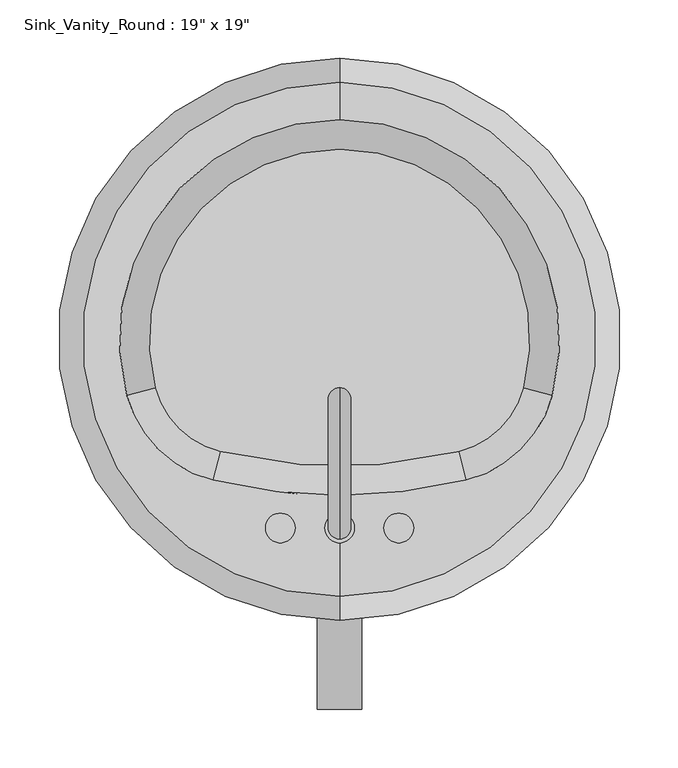
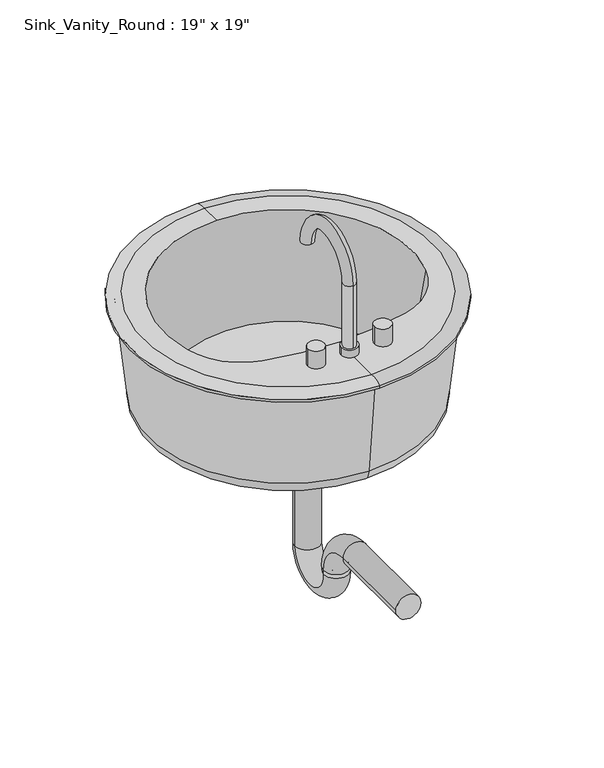
"""IFC4 building model written with IfcOpenShell, lengths in millimetres: flow terminal geometry."""

import ifcopenshell
import ifcopenshell.guid

model = None  # the IFC model being written
_history = None  # IfcOwnerHistory: only IFC2X3 demands one
_inside = {}  # id of a spatial element -> (the spatial element, [elements in it])
_under = {}  # id of a project, library or spatial element -> (it, [spatial elements below it])
_declared = {}  # id of a project -> (the project, [libraries it declares])
_typed = {}  # id of a type object -> (the type object, [elements of that type])
_made_of = {}  # id of a material, layer set ... -> (it, [elements and type objects made of it])


def new_model(schema):
    """Start an empty IFC model of exactly this schema.

    Asked for "IFC4X3", IfcOpenShell would pick the latest addendum, in which some entities
    have other attributes; the version numbers below select the first issue.
    IFC2X3 requires an IfcOwnerHistory on every rooted entity: one is made here for all.
    """
    global model, _history
    if schema == "IFC4X3":
        model = ifcopenshell.file(schema_version=(4, 3, 0, 0))
    else:
        model = ifcopenshell.file(schema=schema)
    _inside.clear()
    _under.clear()
    _declared.clear()
    _typed.clear()
    _made_of.clear()
    _history = None
    if model.schema == "IFC2X3":
        org = make("IfcOrganization", Name="unknown")
        user = make(
            "IfcPersonAndOrganization",
            ThePerson=make("IfcPerson", FamilyName="unknown"),
            TheOrganization=org,
        )
        app = make(
            "IfcApplication",
            ApplicationDeveloper=org,
            Version="unknown",
            ApplicationFullName="unknown",
            ApplicationIdentifier="unknown",
        )
        _history = make(
            "IfcOwnerHistory",
            OwningUser=user,
            OwningApplication=app,
            ChangeAction="ADDED",
            CreationDate=0,
        )
    return model


def make(cls, **values):
    """One entity of the class cls with the attributes given. An attribute that is None is left unset."""
    return model.create_entity(
        cls, **{name: value for name, value in values.items() if value is not None}
    )


def rooted(cls, **values):
    """An entity with a GlobalId (a new one), such as an element, a storey or a relation."""
    return make(cls, GlobalId=ifcopenshell.guid.new(), OwnerHistory=_history, **values)


def si_unit(unit_type, name, prefix=None):
    """IfcSIUnit, for example si_unit("LENGTHUNIT", "METRE", prefix="MILLI")."""
    return make("IfcSIUnit", UnitType=unit_type, Prefix=prefix, Name=name)


def assignment(units):
    """IfcUnitAssignment: the units of a project."""
    return None if units is None else make("IfcUnitAssignment", Units=units)


def point(xyz):
    """IfcCartesianPoint."""
    return None if xyz is None else make("IfcCartesianPoint", Coordinates=xyz)


def direction(xyz):
    """IfcDirection."""
    return None if xyz is None else make("IfcDirection", DirectionRatios=xyz)


def frame(location, z_axis=None, x_axis=None):
    """IfcAxis2Placement3D, a coordinate frame: its origin and axes. An axis left out is left unset."""
    return make(
        "IfcAxis2Placement3D",
        Location=point(location),
        Axis=direction(z_axis),
        RefDirection=direction(x_axis),
    )


def frame_2d(location, x_axis=None):
    """IfcAxis2Placement2D, a coordinate frame in the plane: its origin and x axis."""
    return make(
        "IfcAxis2Placement2D", Location=point(location), RefDirection=direction(x_axis)
    )


def origin():
    """The frame at (0, 0, 0) with its axes left unset."""
    return frame((0.0, 0.0, 0.0))


def place(relative_to, where):
    """IfcLocalPlacement: puts the frame where relative to a parent placement (None: the world)."""
    return make(
        "IfcLocalPlacement", PlacementRelTo=relative_to, RelativePlacement=where
    )


def context(
    kind, dimensions, precision=None, world=None, true_north=None, identifier=None
):
    """IfcGeometricRepresentationContext, for example the 3D "Model" context."""
    return make(
        "IfcGeometricRepresentationContext",
        ContextIdentifier=identifier,
        ContextType=kind,
        CoordinateSpaceDimension=dimensions,
        Precision=precision,
        WorldCoordinateSystem=world,
        TrueNorth=true_north,
    )


def project(units=None, contexts=None):
    """IfcProject with its units and contexts."""
    return rooted(
        "IfcProject",
        Name="project",
        RepresentationContexts=contexts,
        UnitsInContext=assignment(units),
    )


def spatial(cls, under=None, at=None, **own):
    """A site, building, storey or space (cls), placed at a placement, below another one or the project."""
    s = rooted(cls, ObjectPlacement=at, **own)
    if under is not None:
        _under.setdefault(under.id(), (under, []))[1].append(s)
    return s


def polyline(points):
    """IfcPolyline through the points."""
    return make("IfcPolyline", Points=[point(p) for p in points])


def circle_curve(where, radius):
    """IfcCircle in the frame where."""
    return make("IfcCircle", Position=where, Radius=radius)


def ellipse_curve(where, semi_axis1, semi_axis2):
    """IfcEllipse in the frame where."""
    return make(
        "IfcEllipse", Position=where, SemiAxis1=semi_axis1, SemiAxis2=semi_axis2
    )


def trimmed(basis, trim1, trim2, sense, master):
    """IfcTrimmedCurve: the piece of a basis curve between two trims."""
    return make(
        "IfcTrimmedCurve",
        BasisCurve=basis,
        Trim1=trim1,
        Trim2=trim2,
        SenseAgreement=sense,
        MasterRepresentation=master,
    )


def segment(curve, same_sense, transition):
    """IfcCompositeCurveSegment."""
    return make(
        "IfcCompositeCurveSegment",
        Transition=transition,
        SameSense=same_sense,
        ParentCurve=curve,
    )


def composite_curve(segments, self_intersect=None):
    """IfcCompositeCurve: segments joined end to end."""
    return make("IfcCompositeCurve", Segments=segments, SelfIntersect=self_intersect)


def outline(outer, holes=None, kind="AREA"):
    """IfcArbitraryClosedProfileDef: a profile drawn as a closed curve; with holes, ...WithVoids."""
    if holes is None:
        return make("IfcArbitraryClosedProfileDef", ProfileType=kind, OuterCurve=outer)
    return make(
        "IfcArbitraryProfileDefWithVoids",
        ProfileType=kind,
        OuterCurve=outer,
        InnerCurves=holes,
    )


def extrude(swept, where, along, depth):
    """IfcExtrudedAreaSolid: the profile swept, set in the frame where, extruded along a direction by depth."""
    return make(
        "IfcExtrudedAreaSolid",
        SweptArea=swept,
        Position=where,
        ExtrudedDirection=direction(along),
        Depth=depth,
    )


def shape(context_of_items, identifier, shape_type, items):
    """IfcShapeRepresentation: the items that make up one representation, for example the "Body"."""
    return make(
        "IfcShapeRepresentation",
        ContextOfItems=context_of_items,
        RepresentationIdentifier=identifier,
        RepresentationType=shape_type,
        Items=items,
    )


def source(mapping_origin, context_of_items, identifier, shape_type, items):
    """IfcRepresentationMap: a shape defined once, which mapped items show again and again."""
    return make(
        "IfcRepresentationMap",
        MappingOrigin=mapping_origin,
        MappedRepresentation=shape(context_of_items, identifier, shape_type, items),
    )


def transform(
    local_origin,
    x_axis=None,
    y_axis=None,
    z_axis=None,
    scale=None,
    scale2=None,
    scale3=None,
    uniform=True,
):
    """IfcCartesianTransformationOperator3D, or its non-uniform kind. x_axis, y_axis, z_axis: its Axis1, 2, 3."""
    if uniform:
        return make(
            "IfcCartesianTransformationOperator3D",
            Axis1=direction(x_axis),
            Axis2=direction(y_axis),
            LocalOrigin=point(local_origin),
            Scale=scale,
            Axis3=direction(z_axis),
        )
    return make(
        "IfcCartesianTransformationOperator3DnonUniform",
        Axis1=direction(x_axis),
        Axis2=direction(y_axis),
        LocalOrigin=point(local_origin),
        Scale=scale,
        Axis3=direction(z_axis),
        Scale2=scale2,
        Scale3=scale3,
    )


def mapped(mapping_source, mapping_target):
    """IfcMappedItem: shows the shape of a source again, moved by a transform."""
    return make(
        "IfcMappedItem", MappingSource=mapping_source, MappingTarget=mapping_target
    )


def made_of(thing, what):
    """Note that an element or type object is made of a material, layer set ...; save() writes the relation."""
    if what is not None:
        _made_of.setdefault(what.id(), (what, []))[1].append(thing)
    return thing


def element(
    cls,
    number,
    at=None,
    inside=None,
    cuts=None,
    type_object=None,
    material=None,
    context=None,
    identifier="Body",
    shape_type=None,
    held_by="IfcProductDefinitionShape",
    body=None,
    shapes=None,
    **own,
):
    """One element of the class cls, such as IfcWall. Its Tag is "e" and its number.

    at: its placement. inside: the storey or other place that contains it. cuts: it is an
    opening in that element (IfcRelVoidsElement). A single representation is given by context,
    identifier, shape_type and body (its items); several are given by shapes. held_by: the class
    of the entity that holds the representations. save() writes the other relations.
    """
    e = rooted(cls, Tag="e%d" % number, ObjectPlacement=at, **own)
    if body is not None:
        shapes = [shape(context, identifier, shape_type, body)]
    if shapes is not None:
        e.Representation = make(held_by, Representations=shapes)
    if inside is not None:
        _inside.setdefault(inside.id(), (inside, []))[1].append(e)
    if cuts is not None:
        rooted(
            "IfcRelVoidsElement", RelatingBuildingElement=cuts, RelatedOpeningElement=e
        )
    if type_object is not None:
        _typed.setdefault(type_object.id(), (type_object, []))[1].append(e)
    return made_of(e, material)


def aggregate(whole, parts):
    """IfcRelAggregates: a whole, such as a stair, and the parts it consists of."""
    return rooted("IfcRelAggregates", RelatingObject=whole, RelatedObjects=parts)


def save(model, path):
    """Write the relations noted so far, then the file.

    IfcRelAggregates (storeys below a building ...), IfcRelContainedInSpatialStructure (elements
    in a storey), IfcRelDefinesByType, IfcRelAssociatesMaterial and IfcRelDeclares: one each for
    every whole, place, type object, material and project.
    """
    for whole, parts in _under.values():
        aggregate(whole, parts)
    for where, things in _inside.values():
        rooted(
            "IfcRelContainedInSpatialStructure",
            RelatedElements=things,
            RelatingStructure=where,
        )
    for kind, things in _typed.values():
        rooted("IfcRelDefinesByType", RelatedObjects=things, RelatingType=kind)
    for what, things in _made_of.values():
        rooted("IfcRelAssociatesMaterial", RelatedObjects=things, RelatingMaterial=what)
    for by, libraries in _declared.values():
        rooted("IfcRelDeclares", RelatingContext=by, RelatedDefinitions=libraries)
    model.write(path)


def plane_surface(at):
    """IfcPlane: the flat surface through the origin of the frame at, square to its z axis."""
    return make("IfcPlane", Position=at)


def cylinder_surface(at, radius):
    """IfcCylindricalSurface: all points at the distance radius from the z axis of the frame at."""
    return make("IfcCylindricalSurface", Position=at, Radius=radius)


def revolved_surface(curve, axis_point, axis_direction):
    """IfcSurfaceOfRevolution: the curve turned about the line through axis_point along axis_direction."""
    return make(
        "IfcSurfaceOfRevolution",
        SweptCurve=make("IfcArbitraryOpenProfileDef", ProfileType="CURVE", Curve=curve),
        AxisPosition=make("IfcAxis1Placement", Location=point(axis_point), Axis=direction(axis_direction)),
    )


def advanced_brep(points, edges, surfaces, faces):
    """IfcAdvancedBrep: a solid bounded by faces that lie on surfaces and meet in shared edges.

    An edge is (start, end): straight between two places in points (the first is 0);
    or (start, end, curve); or (start, end, curve, False) where it runs against its curve.
    A face is (place in surfaces, loops), or (place, loops, False) where it looks against
    its surface's normal. A loop lists edges by number (the first is 1), with a minus sign
    where the edge is run from its end to its start. The first loop is the outer one.
    """
    corners = [point(p) for p in points]
    vertices = [make("IfcVertexPoint", VertexGeometry=c) for c in corners]
    made = []
    for start, end, *more in edges:
        made.append(
            make(
                "IfcEdgeCurve",
                EdgeStart=vertices[start],
                EdgeEnd=vertices[end],
                EdgeGeometry=more[0] if more else make("IfcPolyline", Points=[corners[start], corners[end]]),
                SameSense=more[1] if len(more) > 1 else True,
            )
        )
    hull = []
    for where, loops, *sense in faces:
        bounds = []
        for j, loop in enumerate(loops):
            ring = [make("IfcOrientedEdge", EdgeElement=made[abs(k) - 1], Orientation=k > 0) for k in loop]
            bounds.append(
                make(
                    "IfcFaceOuterBound" if j == 0 else "IfcFaceBound",
                    Bound=make("IfcEdgeLoop", EdgeList=ring),
                    Orientation=True,
                )
            )
        hull.append(make("IfcAdvancedFace", Bounds=bounds, FaceSurface=surfaces[where], SameSense=sense[0] if sense else True))
    return make("IfcAdvancedBrep", Outer=make("IfcClosedShell", CfsFaces=hull))


def flow_terminal_2c73b8fd(model_context):
    return source(origin(), model_context, "Body", "SolidModel", [
        advanced_brep(
        [(96.6517406, 135.3870093, 796.925), (96.6517406, 156.1322815, 791.36875), (96.6517406, -326.4677185, 791.36875), (96.6517406, -305.7224463, 796.925), (96.6517406, -219.2662048, 796.925), (-11.972132, -206.0284961, 796.925), (-85.8055572, -133.3356834, 796.925), (96.6517406, 103.5405705, 796.925), (279.1090383, -133.3356834, 796.925), (205.2756132, -206.0284961, 796.925), (96.6517406, 107.1264028, 615.95), (96.6517406, -85.1677185, 615.95), (96.6517406, -277.4618398, 615.95), (96.6517406, -298.0181731, 637.1342611), (96.6517406, 127.6827361, 637.1342611), (96.6517406, -314.5614685, 787.4), (96.6517406, 144.2260315, 787.4), (96.6517406, -326.4677185, 787.4), (96.6517406, 156.1322815, 787.4), (-61.2469361, -126.85231, 635.0), (-5.8718673, -181.3719195, 635.0), (199.1753484, -181.3719195, 635.0), (254.5504173, -126.85231, 635.0)],
        [
            (0, 1, circle_curve(frame((96.6517406, 139.1020246, 769.289434), z_axis=(-1.0, 0.0, 0.0), x_axis=(0.0, 1.0, 0.0)), 27.8841505)),
            (1, 2, circle_curve(frame((96.6517406, -85.1677185, 791.36875), z_axis=(0.0, 0.0, 1.0), x_axis=(0.0, -1.0, 0.0)), 241.3)),
            (2, 3, circle_curve(frame((96.6517406, -309.4374616, 769.289434), z_axis=(-1.0, 0.0, 0.0), x_axis=(0.0, -1.0, 0.0)), 27.8841505)),
            (3, 0, circle_curve(frame((96.6517406, -85.1677185, 796.925), z_axis=(0.0, 0.0, -1.0), x_axis=(0.0, -1.0, 0.0)), 220.5547278)),
            (2, 1, circle_curve(frame((96.6517406, -85.1677185, 791.36875), z_axis=(0.0, 0.0, 1.0), x_axis=(0.0, -1.0, 0.0)), 241.3)),
            (0, 3, circle_curve(frame((96.6517406, -85.1677185, 796.925), z_axis=(0.0, 0.0, -1.0), x_axis=(0.0, -1.0, 0.0)), 220.5547278)),
            (3, 4),
            (4, 5, circle_curve(frame((96.6517406, 233.0168462, 796.925), z_axis=(0.0, 0.0, -1.0), x_axis=(-0.24016790448601874, -0.9707313622495126, 0.0)), 452.283051)),
            (5, 6, circle_curve(frame((12.4289271, -107.4021897, 796.925), z_axis=(0.0, 0.0, -1.0), x_axis=(-0.9668748453196011, -0.25525092260008997, 0.0)), 101.6)),
            (6, 7, circle_curve(frame((96.6517406, -85.1677185, 796.925), z_axis=(0.0, 0.0, -1.0), x_axis=(0.9668748453195979, -0.2552509226001031, 0.0)), 188.708289)),
            (7, 0),
            (7, 8, circle_curve(frame((96.6517406, -85.1677185, 796.925), z_axis=(0.0, 0.0, -1.0), x_axis=(0.9668748453195979, -0.2552509226001031, 0.0)), 188.708289)),
            (8, 9, circle_curve(frame((180.8745541, -107.4021897, 796.925), z_axis=(0.0, 0.0, -1.0), x_axis=(0.2401679044860015, -0.970731362249517, 0.0)), 101.6)),
            (9, 4, circle_curve(frame((96.6517406, 233.0168462, 796.925), z_axis=(0.0, 0.0, -1.0), x_axis=(-0.24016790448601874, -0.9707313622495126, 0.0)), 452.283051)),
            (10, 11),
            (11, 12),
            (12, 10, circle_curve(frame((96.6517406, -85.1677185, 615.95), z_axis=(0.0, 0.0, -1.0), x_axis=(0.0, -1.0, 0.0)), 192.2941213)),
            (10, 12, circle_curve(frame((96.6517406, -85.1677185, 615.95), z_axis=(0.0, 0.0, -1.0), x_axis=(0.0, -1.0, 0.0)), 192.2941213)),
            (12, 13, circle_curve(frame((96.6517406, -277.4618398, 636.5156396), z_axis=(-1.0, 0.0, 0.0), x_axis=(0.0, -1.0, 0.0)), 20.5656396)),
            (13, 14, circle_curve(frame((96.6517406, -85.1677185, 637.1342611), z_axis=(0.0, 0.0, -1.0), x_axis=(0.0, -1.0, 0.0)), 212.8504546)),
            (14, 10, circle_curve(frame((96.6517406, 107.1264028, 636.5156396), z_axis=(-1.0, 0.0, 0.0), x_axis=(0.0, 1.0, 0.0)), 20.5656396)),
            (14, 13, circle_curve(frame((96.6517406, -85.1677185, 637.1342611), z_axis=(0.0, 0.0, -1.0), x_axis=(0.0, -1.0, 0.0)), 212.8504546)),
            (13, 15),
            (15, 16, circle_curve(frame((96.6517406, -85.1677185, 787.4), z_axis=(0.0, 0.0, -1.0), x_axis=(0.0, -1.0, 0.0)), 229.39375)),
            (16, 14),
            (16, 15, circle_curve(frame((96.6517406, -85.1677185, 787.4), z_axis=(0.0, 0.0, -1.0), x_axis=(0.0, -1.0, 0.0)), 229.39375)),
            (15, 17),
            (17, 18, circle_curve(frame((96.6517406, -85.1677185, 787.4), z_axis=(0.0, 0.0, -1.0), x_axis=(0.0, -1.0, 0.0)), 241.3)),
            (18, 16),
            (18, 17, circle_curve(frame((96.6517406, -85.1677185, 787.4), z_axis=(0.0, 0.0, -1.0), x_axis=(0.0, -1.0, 0.0)), 241.3)),
            (1, 18),
            (17, 2),
            (19, 20, circle_curve(frame((12.4289271, -107.4021897, 635.0), z_axis=(0.0, 0.0, 1.0), x_axis=(-0.9668748453196011, -0.25525092260008997, 0.0)), 76.2)),
            (20, 21, circle_curve(frame((96.6517406, 233.0168462, 635.0), z_axis=(0.0, 0.0, 1.0), x_axis=(-0.24016790448601874, -0.9707313622495126, 0.0)), 426.883051)),
            (21, 22, circle_curve(frame((180.8745541, -107.4021897, 635.0), z_axis=(0.0, 0.0, 1.0), x_axis=(0.2401679044860015, -0.970731362249517, 0.0)), 76.2)),
            (22, 19, circle_curve(frame((96.6517406, -85.1677185, 635.0), z_axis=(0.0, 0.0, 1.0), x_axis=(0.9668748453195979, -0.2552509226001031, 0.0)), 163.308289)),
            (19, 6),
            (5, 20),
            (9, 21),
            (8, 22),
        ],
        [
            revolved_surface(trimmed(ellipse_curve(frame((96.6517406, -309.4374616, 769.289434), z_axis=(-1.0, 0.0, 0.0), x_axis=(0.0, -1.0, 0.0)), 27.8841505, 27.8841505), [point((96.6517406, -326.4677185, 791.36875))], [point((96.6517406, -305.7224463, 796.925))], True, "CARTESIAN"), (96.6517406, -85.1677185, 796.925), (0.0, 0.0, 1.0)),
            plane_surface(frame((96.6517406, -85.1677185, 796.925), z_axis=(0.0, 0.0, 1.0), x_axis=(0.0, -1.0, 0.0))),
            plane_surface(frame((96.6517406, -85.1677185, 615.95), z_axis=(0.0, 0.0, -1.0), x_axis=(0.0, -1.0, 0.0))),
            revolved_surface(trimmed(ellipse_curve(frame((96.6517406, -277.4618398, 636.5156396), z_axis=(-1.0, 0.0, 0.0), x_axis=(0.0, -1.0, 0.0)), 20.5656396, 20.5656396), [point((96.6517406, -277.4618398, 615.95))], [point((96.6517406, -298.0181731, 637.1342611))], True, "CARTESIAN"), (96.6517406, -85.1677185, 796.925), (0.0, 0.0, 1.0)),
            revolved_surface(polyline([(96.6517406, -298.0181731, 637.1342611), (96.6517406, -314.5614685, 787.4)]), (96.6517406, -85.1677185, 796.925), (0.0, 0.0, 1.0)),
            plane_surface(frame((96.6517406, -85.1677185, 787.4), z_axis=(0.0, 0.0, -1.0), x_axis=(0.0, -1.0, 0.0))),
            cylinder_surface(frame((96.6517406, -85.1677185, 796.925), z_axis=(0.0, 0.0, 1.0), x_axis=(0.0, -1.0, 0.0)), 241.3),
            plane_surface(frame((96.6517406, -154.1121147, 635.0), z_axis=(0.0, 0.0, 1.0), x_axis=(-0.2552509226000978, 0.9668748453195992, 0.0))),
            revolved_surface(polyline([(-85.8055572, -133.3356834, 796.925), (-61.246936125000005, -126.852309975, 635.0)]), (12.4289271, -107.4021897, 149.225), (0.0, 0.0, 1.0)),
            revolved_surface(polyline([(-11.972132000000002, -206.0284961, 796.9250000000002), (-5.871867225621074, -181.3719194941331, 635.0)]), (96.6517406, 233.0168462, -2086.3794501), (0.0, 0.0, 1.0)),
            revolved_surface(polyline([(205.2756132, -206.0284961, 796.925), (199.175348425, -181.3719195, 635.0)]), (180.8745541, -107.4021897, 149.225), (0.0, 0.0, 1.0)),
            revolved_surface(polyline([(279.1090383, -133.3356834, 796.925), (254.55041724055098, -126.85230996360858, 635.0)]), (96.6517406, -85.1677185, -406.0903427), (0.0, 0.0, 1.0)),
        ],
        [
            (0, [[1, 2, 3, 4]]),
            (0, [[5, -1, 6, -3]]),
            (1, [[7, 8, 9, 10, 11, -4]]),
            (1, [[-11, 12, 13, 14, -7, -6]]),
            (2, [[15, 16, 17]]),
            (2, [[-15, 18, -16]]),
            (3, [[19, 20, 21, -17]]),
            (3, [[-21, 22, -19, -18]]),
            (4, [[23, 24, 25, -20]]),
            (4, [[-25, 26, -23, -22]]),
            (5, [[27, 28, 29, -24]]),
            (5, [[-29, 30, -27, -26]]),
            (6, [[31, -28, 32, -2]]),
            (6, [[-32, -30, -31, -5]]),
            (7, [[33, 34, 35, 36]]),
            (8, [[37, -9, 38, -33]]),
            (9, [[-38, -8, -14, 39, -34]]),
            (10, [[-39, -13, 40, -35]]),
            (11, [[-40, -12, -10, -37, -36]]),
        ],
    ),
        advanced_brep(
        [(83.9517406, -247.0927185, 796.925), (109.3517406, -247.0927185, 796.925), (96.6517406, -237.5677185, 909.6375), (96.6517406, -237.5677185, 809.625), (96.6517406, -256.6177185, 809.625), (96.6517406, -256.6177185, 909.6375), (96.6517406, -145.7775038, 909.6375), (96.6517406, -126.7275038, 909.6375), (83.9517406, -247.0927185, 809.625), (109.3517406, -247.0927185, 809.625)],
        [
            (0, 1, circle_curve(frame((96.6517406, -247.0927185, 796.925), z_axis=(0.0, 0.0, -1.0), x_axis=(1.0, 0.0, 0.0)), 12.7)),
            (1, 0, circle_curve(frame((96.6517406, -247.0927185, 796.925), z_axis=(0.0, 0.0, -1.0), x_axis=(1.0, 0.0, 0.0)), 12.7)),
            (2, 3),
            (3, 4, circle_curve(frame((96.6517406, -247.0927185, 809.625), z_axis=(0.0, 0.0, 1.0), x_axis=(0.0, -1.0, 0.0)), 9.525)),
            (4, 5),
            (5, 2, circle_curve(frame((96.6517406, -247.0927185, 909.6375), z_axis=(0.0, 0.0, -1.0), x_axis=(0.0, -1.0, 0.0)), 9.525)),
            (4, 3, circle_curve(frame((96.6517406, -247.0927185, 809.625), z_axis=(0.0, 0.0, 1.0), x_axis=(0.0, -1.0, 0.0)), 9.525)),
            (2, 5, circle_curve(frame((96.6517406, -247.0927185, 909.6375), z_axis=(0.0, 0.0, -1.0), x_axis=(0.0, -1.0, 0.0)), 9.525)),
            (6, 7, circle_curve(frame((96.6517406, -136.2525038, 909.6375), z_axis=(0.0, 0.0, -1.0), x_axis=(0.0, 1.0, 0.0)), 9.525)),
            (7, 6, circle_curve(frame((96.6517406, -136.2525038, 909.6375), z_axis=(0.0, 0.0, -1.0), x_axis=(0.0, 1.0, 0.0)), 9.525)),
            (5, 7, circle_curve(frame((96.6517406, -191.6726112, 909.6375), z_axis=(-1.0, 0.0, 0.0), x_axis=(0.0, -1.0, 0.0)), 64.9451073)),
            (6, 2, circle_curve(frame((96.6517406, -191.6726112, 909.6375), z_axis=(1.0, 0.0, 0.0), x_axis=(0.0, -1.0, 0.0)), 45.8951073)),
            (8, 9, circle_curve(frame((96.6517406, -247.0927185, 809.625), z_axis=(0.0, 0.0, 1.0), x_axis=(1.0, 0.0, 0.0)), 12.7)),
            (9, 8, circle_curve(frame((96.6517406, -247.0927185, 809.625), z_axis=(0.0, 0.0, 1.0), x_axis=(1.0, 0.0, 0.0)), 12.7)),
            (9, 1),
            (0, 8),
        ],
        [
            plane_surface(frame((96.6517406, -237.5677185, 796.925), z_axis=(0.0, 0.0, -1.0), x_axis=(1.0, 0.0, 0.0))),
            cylinder_surface(frame((96.6517406, -247.0927185, 796.925), z_axis=(0.0, 0.0, -1.0), x_axis=(0.0, -1.0, 0.0)), 9.525),
            plane_surface(frame((96.6517406, -191.6726112, 909.6375), z_axis=(0.0, 0.0, -1.0), x_axis=(0.0, 1.0, 0.0))),
            revolved_surface(trimmed(ellipse_curve(frame((96.6517406, -247.0927185, 909.6375), z_axis=(0.0, 0.0, 1.0), x_axis=(0.0, -1.0, 0.0)), 9.525, 9.525), [point((96.6517406, -237.5677185, 909.6375))], [point((96.6517406, -256.6177185, 909.6375))], True, "CARTESIAN"), (96.6517406, -191.6726112, 909.6375), (1.0, 0.0, 0.0)),
            revolved_surface(trimmed(ellipse_curve(frame((96.6517406, -247.0927185, 909.6375), z_axis=(0.0, 0.0, 1.0), x_axis=(0.0, -1.0, 0.0)), 9.525, 9.525), [point((96.6517406, -256.6177185, 909.6375))], [point((96.6517406, -237.5677185, 909.6375))], True, "CARTESIAN"), (96.6517406, -191.6726112, 909.6375), (1.0, 0.0, 0.0)),
            plane_surface(frame((109.3517406, -247.0927185, 809.625), z_axis=(0.0, 0.0, 1.0), x_axis=(0.0, -1.0, 0.0))),
            cylinder_surface(frame((96.6517406, -247.0927185, 796.925), z_axis=(0.0, 0.0, 1.0), x_axis=(1.0, 0.0, 0.0)), 12.7),
        ],
        [
            (0, [[1, 2]]),
            (1, [[3, 4, 5, 6]]),
            (1, [[-5, 7, -3, 8]]),
            (2, [[9, 10]]),
            (3, [[11, -9, 12, -6]]),
            (4, [[-12, -10, -11, -8]]),
            (5, [[13, 14], [-7, -4]]),
            (6, [[15, -1, 16, -14]]),
            (6, [[-16, -2, -15, -13]]),
        ],
    ),
        extrude(outline(composite_curve([segment(trimmed(circle_curve(frame_2d((45.8517406, -247.0927185)), 12.7), [point((33.1517406, -247.0927185))], [point((58.5517406, -247.0927185))], False, "CARTESIAN"), True, "CONTINUOUS"), segment(trimmed(circle_curve(frame_2d((45.8517406, -247.0927185)), 12.7), [point((58.5517406, -247.0927185))], [point((33.1517406, -247.0927185))], False, "CARTESIAN"), True, "CONTINUOUS")], self_intersect=False)), frame((0.0, 0.0, 796.925), z_axis=(0.0, 0.0, 1.0), x_axis=(1.0, 0.0, 0.0)), (0.0, 0.0, 1.0), 28.575),
        extrude(outline(composite_curve([segment(trimmed(circle_curve(frame_2d((147.4517406, -247.0927185)), 12.7), [point((134.7517406, -247.0927185))], [point((160.1517406, -247.0927185))], False, "CARTESIAN"), True, "CONTINUOUS"), segment(trimmed(circle_curve(frame_2d((147.4517406, -247.0927185)), 12.7), [point((160.1517406, -247.0927185))], [point((134.7517406, -247.0927185))], False, "CARTESIAN"), True, "CONTINUOUS")], self_intersect=False)), frame((0.0, 0.0, 796.925), z_axis=(0.0, 0.0, 1.0), x_axis=(1.0, 0.0, 0.0)), (0.0, 0.0, 1.0), 28.575),
        advanced_brep(
        [(77.6017406, -135.9677185, 615.95), (115.7017406, -135.9677185, 615.95), (115.7017406, -135.9677185, 425.45), (77.6017406, -135.9677185, 425.45), (115.7017406, -212.1677185, 425.45), (77.6017406, -212.1677185, 425.45), (115.7017406, -212.1677185, 431.8), (77.6017406, -212.1677185, 431.8), (115.7017406, -262.9677185, 482.6), (77.6017406, -262.9677185, 482.6), (77.6017406, -402.6677185, 482.6), (115.7017406, -402.6677185, 482.6)],
        [
            (0, 1, circle_curve(frame((96.6517406, -135.9677185, 615.95), z_axis=(0.0, 0.0, 1.0), x_axis=(1.0, 0.0, 0.0)), 19.05)),
            (1, 0, circle_curve(frame((96.6517406, -135.9677185, 615.95), z_axis=(0.0, 0.0, 1.0), x_axis=(1.0, 0.0, 0.0)), 19.05)),
            (1, 2),
            (2, 3, circle_curve(frame((96.6517406, -135.9677185, 425.45), z_axis=(0.0, 0.0, 1.0), x_axis=(1.0, 0.0, 0.0)), 19.05)),
            (3, 0),
            (3, 2, circle_curve(frame((96.6517406, -135.9677185, 425.45), z_axis=(0.0, 0.0, 1.0), x_axis=(1.0, 0.0, 0.0)), 19.05)),
            (4, 5, circle_curve(frame((96.6517406, -212.1677185, 425.45), z_axis=(0.0, 0.0, -1.0), x_axis=(1.0, 0.0, 0.0)), 19.05)),
            (5, 3, circle_curve(frame((77.6017406, -174.0677185, 425.45), z_axis=(1.0, 0.0, 0.0), x_axis=(0.0, 1.0, 0.0)), 38.1)),
            (2, 4, circle_curve(frame((115.7017406, -174.0677185, 425.45), z_axis=(-1.0, 0.0, 0.0), x_axis=(0.0, 1.0, 0.0)), 38.1)),
            (5, 4, circle_curve(frame((96.6517406, -212.1677185, 425.45), z_axis=(0.0, 0.0, -1.0), x_axis=(1.0, 0.0, 0.0)), 19.05)),
            (4, 6),
            (6, 7, circle_curve(frame((96.6517406, -212.1677185, 431.8), z_axis=(0.0, 0.0, -1.0), x_axis=(1.0, 0.0, 0.0)), 19.05)),
            (7, 5),
            (7, 6, circle_curve(frame((96.6517406, -212.1677185, 431.8), z_axis=(0.0, 0.0, -1.0), x_axis=(1.0, 0.0, 0.0)), 19.05)),
            (8, 9, circle_curve(frame((96.6517406, -262.9677185, 482.6), z_axis=(0.0, 1.0, 0.0), x_axis=(1.0, 0.0, 0.0)), 19.05)),
            (9, 7, circle_curve(frame((77.6017406, -262.9677185, 431.8), z_axis=(-1.0, 0.0, 0.0), x_axis=(0.0, 1.0, 0.0)), 50.8)),
            (6, 8, circle_curve(frame((115.7017406, -262.9677185, 431.8), z_axis=(1.0, 0.0, 0.0), x_axis=(0.0, 1.0, 0.0)), 50.8)),
            (9, 8, circle_curve(frame((96.6517406, -262.9677185, 482.6), z_axis=(0.0, 1.0, 0.0), x_axis=(1.0, 0.0, 0.0)), 19.05)),
            (10, 11, circle_curve(frame((96.6517406, -402.6677185, 482.6), z_axis=(0.0, -1.0, 0.0), x_axis=(1.0, 0.0, 0.0)), 19.05)),
            (11, 10, circle_curve(frame((96.6517406, -402.6677185, 482.6), z_axis=(0.0, -1.0, 0.0), x_axis=(1.0, 0.0, 0.0)), 19.05)),
            (8, 11),
            (10, 9),
        ],
        [
            plane_surface(frame((96.6517406, -135.9677185, 615.95), z_axis=(0.0, 0.0, 1.0), x_axis=(1.0, 0.0, 0.0))),
            cylinder_surface(frame((96.6517406, -135.9677185, 615.95), z_axis=(0.0, 0.0, 1.0), x_axis=(1.0, 0.0, 0.0)), 19.05),
            revolved_surface(trimmed(ellipse_curve(frame((96.6517406, -135.9677185, 425.45), z_axis=(0.0, 0.0, -1.0), x_axis=(1.0, 0.0, 0.0)), 19.05, 19.05), [point((77.6017406, -135.9677185, 425.45))], [point((115.7017406, -135.9677185, 425.45))], True, "CARTESIAN"), (96.6517406, -174.0677185, 425.45), (1.0, 0.0, 0.0)),
            revolved_surface(trimmed(ellipse_curve(frame((96.6517406, -135.9677185, 425.45), z_axis=(0.0, 0.0, -1.0), x_axis=(1.0, 0.0, 0.0)), 19.05, 19.05), [point((115.7017406, -135.9677185, 425.45))], [point((77.6017406, -135.9677185, 425.45))], True, "CARTESIAN"), (96.6517406, -174.0677185, 425.45), (1.0, 0.0, 0.0)),
            cylinder_surface(frame((96.6517406, -212.1677185, 425.45), z_axis=(0.0, 0.0, -1.0), x_axis=(1.0, 0.0, 0.0)), 19.05),
            revolved_surface(trimmed(ellipse_curve(frame((96.6517406, -212.1677185, 431.8), z_axis=(0.0, 0.0, 1.0), x_axis=(1.0, 0.0, 0.0)), 19.05, 19.05), [point((77.6017406, -212.1677185, 431.8))], [point((115.7017406, -212.1677185, 431.8))], True, "CARTESIAN"), (96.6517406, -262.9677185, 431.8), (-1.0, 0.0, 0.0)),
            revolved_surface(trimmed(ellipse_curve(frame((96.6517406, -212.1677185, 431.8), z_axis=(0.0, 0.0, 1.0), x_axis=(1.0, 0.0, 0.0)), 19.05, 19.05), [point((115.7017406, -212.1677185, 431.8))], [point((77.6017406, -212.1677185, 431.8))], True, "CARTESIAN"), (96.6517406, -262.9677185, 431.8), (-1.0, 0.0, 0.0)),
            plane_surface(frame((96.6517406, -402.6677185, 482.6), z_axis=(0.0, -1.0, 0.0), x_axis=(1.0, 0.0, 0.0))),
            cylinder_surface(frame((96.6517406, -262.9677185, 482.6), z_axis=(0.0, 1.0, 0.0), x_axis=(1.0, 0.0, 0.0)), 19.05),
        ],
        [
            (0, [[1, 2]]),
            (1, [[3, 4, 5, -2]]),
            (1, [[-5, 6, -3, -1]]),
            (2, [[7, 8, -4, 9]]),
            (3, [[10, -9, -6, -8]]),
            (4, [[11, 12, 13, -7]]),
            (4, [[-13, 14, -11, -10]]),
            (5, [[15, 16, -12, 17]]),
            (6, [[18, -17, -14, -16]]),
            (7, [[19, 20]]),
            (8, [[21, -19, 22, -15]]),
            (8, [[-22, -20, -21, -18]]),
        ],
    ),
    ])


if __name__ == "__main__":
    model = new_model("IFC4")
    model_context = context("Model", 3, world=origin())
    ifc_project = project(units=[si_unit("LENGTHUNIT", "METRE", prefix="MILLI")], contexts=[model_context])
    site = spatial("IfcSite", under=ifc_project)
    building = spatial("IfcBuilding", under=site)
    placement = place(None, origin())
    flow_terminal_shape = flow_terminal_2c73b8fd(model_context)
    element("IfcFlowTerminal", 1, ObjectType="Sink_Vanity_Round : 19\" x 19\"", at=placement, inside=building, context=model_context, shape_type="MappedRepresentation", body=[
        mapped(flow_terminal_shape, transform((0.0, 0.0, 0.0), x_axis=(1.0, 0.0, 0.0), y_axis=(0.0, 1.0, 0.0), z_axis=(0.0, 0.0, 1.0))),
    ])
    save(model, "model.ifc")

# Revit data of these elements
# Type "Sink_Vanity_Round : 19\" x 19\""
#   Assembly Code = "D2010400"
#   Top Of Counter = 2' - 7"
#   Basin Material = Fixtures - Porcelain - Linen
#   Faucet Material = Fixtures - Metal - Chrome
# Element 1 (IfcFlowTerminal, "Sink_Vanity_Round : 19\" x 19\"")
#   Materials on its faces: "Fixtures - Metal - Chrome", "Fixtures - Porcelain - Linen"
# Materials
#   "Fixtures - Porcelain - Linen": class "Unassigned", colour RGB 249 239 230, transparency 0, Keynote = "15410", Description = "Porcelain Sinks and Water Closets"
#   "Fixtures - Metal - Chrome": class "Unassigned", colour RGB 247 247 247, transparency 0, Description = "Chrome finished Plumbing Fixtures"
